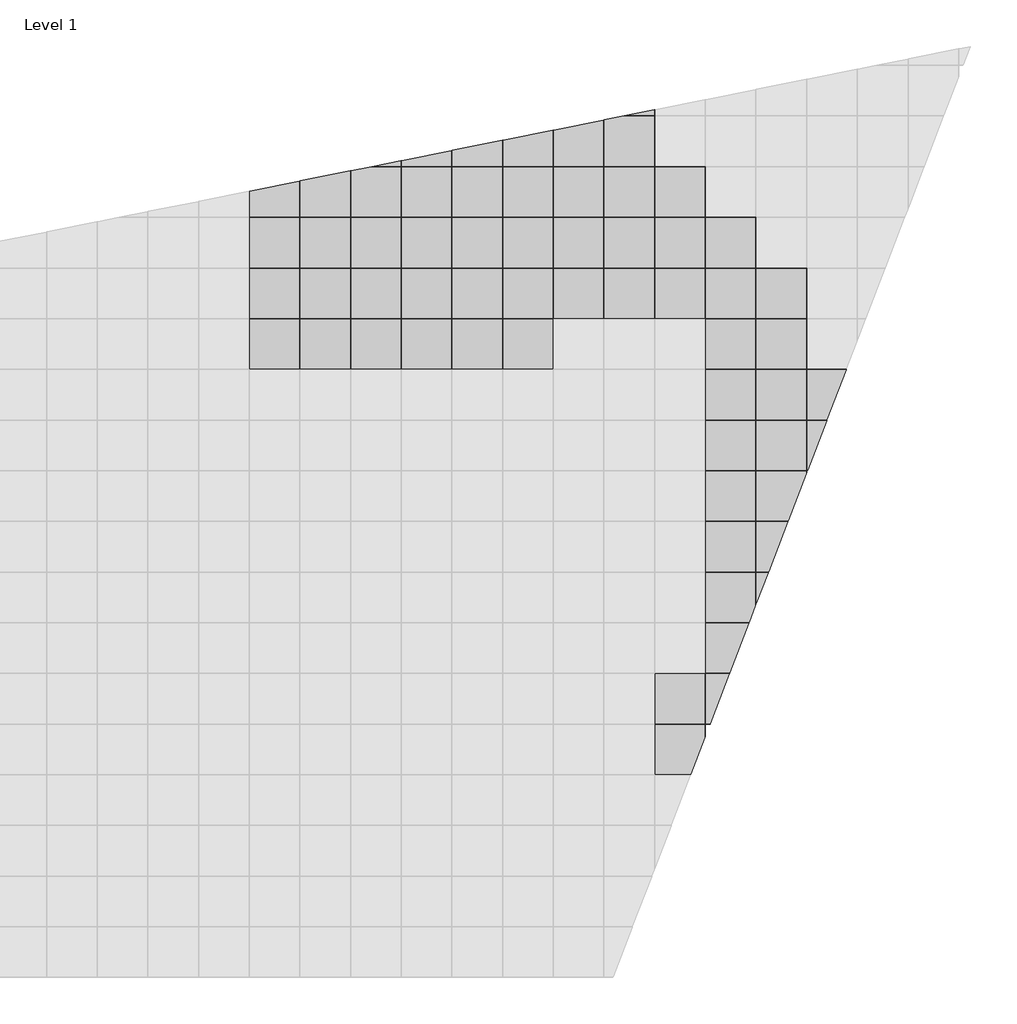
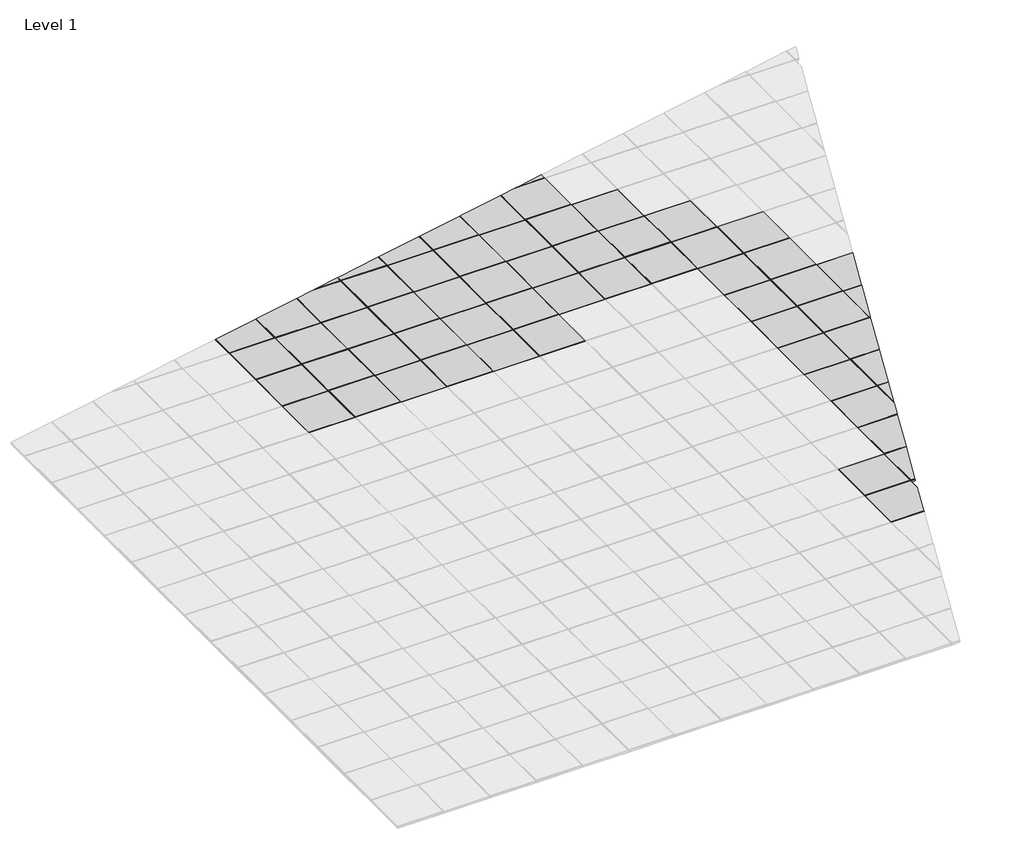
# One storey, part 7 of 18: 61 plates.
"""IFC4 building model written with IfcOpenShell, lengths in millimetres."""

import ifcopenshell
import ifcopenshell.guid

model = None  # the IFC model being written
_history = None  # IfcOwnerHistory: only IFC2X3 demands one
_inside = {}  # id of a spatial element -> (the spatial element, [elements in it])
_under = {}  # id of a project, library or spatial element -> (it, [spatial elements below it])
_declared = {}  # id of a project -> (the project, [libraries it declares])
_typed = {}  # id of a type object -> (the type object, [elements of that type])
_made_of = {}  # id of a material, layer set ... -> (it, [elements and type objects made of it])


def new_model(schema):
    """Start an empty IFC model of exactly this schema.

    Asked for "IFC4X3", IfcOpenShell would pick the latest addendum, in which some entities
    have other attributes; the version numbers below select the first issue.
    IFC2X3 requires an IfcOwnerHistory on every rooted entity: one is made here for all.
    """
    global model, _history
    if schema == "IFC4X3":
        model = ifcopenshell.file(schema_version=(4, 3, 0, 0))
    else:
        model = ifcopenshell.file(schema=schema)
    _inside.clear()
    _under.clear()
    _declared.clear()
    _typed.clear()
    _made_of.clear()
    _history = None
    if model.schema == "IFC2X3":
        org = make("IfcOrganization", Name="unknown")
        user = make(
            "IfcPersonAndOrganization",
            ThePerson=make("IfcPerson", FamilyName="unknown"),
            TheOrganization=org,
        )
        app = make(
            "IfcApplication",
            ApplicationDeveloper=org,
            Version="unknown",
            ApplicationFullName="unknown",
            ApplicationIdentifier="unknown",
        )
        _history = make(
            "IfcOwnerHistory",
            OwningUser=user,
            OwningApplication=app,
            ChangeAction="ADDED",
            CreationDate=0,
        )
    return model


def make(cls, **values):
    """One entity of the class cls with the attributes given. An attribute that is None is left unset."""
    return model.create_entity(
        cls, **{name: value for name, value in values.items() if value is not None}
    )


def rooted(cls, **values):
    """An entity with a GlobalId (a new one), such as an element, a storey or a relation."""
    return make(cls, GlobalId=ifcopenshell.guid.new(), OwnerHistory=_history, **values)


def si_unit(unit_type, name, prefix=None):
    """IfcSIUnit, for example si_unit("LENGTHUNIT", "METRE", prefix="MILLI")."""
    return make("IfcSIUnit", UnitType=unit_type, Prefix=prefix, Name=name)


def assignment(units):
    """IfcUnitAssignment: the units of a project."""
    return None if units is None else make("IfcUnitAssignment", Units=units)


def point(xyz):
    """IfcCartesianPoint."""
    return None if xyz is None else make("IfcCartesianPoint", Coordinates=xyz)


def direction(xyz):
    """IfcDirection."""
    return None if xyz is None else make("IfcDirection", DirectionRatios=xyz)


def frame(location, z_axis=None, x_axis=None):
    """IfcAxis2Placement3D, a coordinate frame: its origin and axes. An axis left out is left unset."""
    return make(
        "IfcAxis2Placement3D",
        Location=point(location),
        Axis=direction(z_axis),
        RefDirection=direction(x_axis),
    )


def origin():
    """The frame at (0, 0, 0) with its axes left unset."""
    return frame((0.0, 0.0, 0.0))


def origin_with_axes():
    """The frame at (0, 0, 0) with the z axis (0, 0, 1) and the x axis (1, 0, 0) written out."""
    return frame((0.0, 0.0, 0.0), z_axis=(0.0, 0.0, 1.0), x_axis=(1.0, 0.0, 0.0))


def place(relative_to, where):
    """IfcLocalPlacement: puts the frame where relative to a parent placement (None: the world)."""
    return make(
        "IfcLocalPlacement", PlacementRelTo=relative_to, RelativePlacement=where
    )


def context(
    kind, dimensions, precision=None, world=None, true_north=None, identifier=None
):
    """IfcGeometricRepresentationContext, for example the 3D "Model" context."""
    return make(
        "IfcGeometricRepresentationContext",
        ContextIdentifier=identifier,
        ContextType=kind,
        CoordinateSpaceDimension=dimensions,
        Precision=precision,
        WorldCoordinateSystem=world,
        TrueNorth=true_north,
    )


def project(units=None, contexts=None):
    """IfcProject with its units and contexts."""
    return rooted(
        "IfcProject",
        Name="project",
        RepresentationContexts=contexts,
        UnitsInContext=assignment(units),
    )


def spatial(cls, under=None, at=None, **own):
    """A site, building, storey or space (cls), placed at a placement, below another one or the project."""
    s = rooted(cls, ObjectPlacement=at, **own)
    if under is not None:
        _under.setdefault(under.id(), (under, []))[1].append(s)
    return s


def polyline(points):
    """IfcPolyline through the points."""
    return make("IfcPolyline", Points=[point(p) for p in points])


def outline(outer, holes=None, kind="AREA"):
    """IfcArbitraryClosedProfileDef: a profile drawn as a closed curve; with holes, ...WithVoids."""
    if holes is None:
        return make("IfcArbitraryClosedProfileDef", ProfileType=kind, OuterCurve=outer)
    return make(
        "IfcArbitraryProfileDefWithVoids",
        ProfileType=kind,
        OuterCurve=outer,
        InnerCurves=holes,
    )


def extrude(swept, where, along, depth):
    """IfcExtrudedAreaSolid: the profile swept, set in the frame where, extruded along a direction by depth."""
    return make(
        "IfcExtrudedAreaSolid",
        SweptArea=swept,
        Position=where,
        ExtrudedDirection=direction(along),
        Depth=depth,
    )


def shape(context_of_items, identifier, shape_type, items):
    """IfcShapeRepresentation: the items that make up one representation, for example the "Body"."""
    return make(
        "IfcShapeRepresentation",
        ContextOfItems=context_of_items,
        RepresentationIdentifier=identifier,
        RepresentationType=shape_type,
        Items=items,
    )


def source(mapping_origin, context_of_items, identifier, shape_type, items):
    """IfcRepresentationMap: a shape defined once, which mapped items show again and again."""
    return make(
        "IfcRepresentationMap",
        MappingOrigin=mapping_origin,
        MappedRepresentation=shape(context_of_items, identifier, shape_type, items),
    )


def transform(
    local_origin,
    x_axis=None,
    y_axis=None,
    z_axis=None,
    scale=None,
    scale2=None,
    scale3=None,
    uniform=True,
):
    """IfcCartesianTransformationOperator3D, or its non-uniform kind. x_axis, y_axis, z_axis: its Axis1, 2, 3."""
    if uniform:
        return make(
            "IfcCartesianTransformationOperator3D",
            Axis1=direction(x_axis),
            Axis2=direction(y_axis),
            LocalOrigin=point(local_origin),
            Scale=scale,
            Axis3=direction(z_axis),
        )
    return make(
        "IfcCartesianTransformationOperator3DnonUniform",
        Axis1=direction(x_axis),
        Axis2=direction(y_axis),
        LocalOrigin=point(local_origin),
        Scale=scale,
        Axis3=direction(z_axis),
        Scale2=scale2,
        Scale3=scale3,
    )


def mapped(mapping_source, mapping_target):
    """IfcMappedItem: shows the shape of a source again, moved by a transform."""
    return make(
        "IfcMappedItem", MappingSource=mapping_source, MappingTarget=mapping_target
    )


def made_of(thing, what):
    """Note that an element or type object is made of a material, layer set ...; save() writes the relation."""
    if what is not None:
        _made_of.setdefault(what.id(), (what, []))[1].append(thing)
    return thing


def element(
    cls,
    number,
    at=None,
    inside=None,
    cuts=None,
    type_object=None,
    material=None,
    context=None,
    identifier="Body",
    shape_type=None,
    held_by="IfcProductDefinitionShape",
    body=None,
    shapes=None,
    **own,
):
    """One element of the class cls, such as IfcWall. Its Tag is "e" and its number.

    at: its placement. inside: the storey or other place that contains it. cuts: it is an
    opening in that element (IfcRelVoidsElement). A single representation is given by context,
    identifier, shape_type and body (its items); several are given by shapes. held_by: the class
    of the entity that holds the representations. save() writes the other relations.
    """
    e = rooted(cls, Tag="e%d" % number, ObjectPlacement=at, **own)
    if body is not None:
        shapes = [shape(context, identifier, shape_type, body)]
    if shapes is not None:
        e.Representation = make(held_by, Representations=shapes)
    if inside is not None:
        _inside.setdefault(inside.id(), (inside, []))[1].append(e)
    if cuts is not None:
        rooted(
            "IfcRelVoidsElement", RelatingBuildingElement=cuts, RelatedOpeningElement=e
        )
    if type_object is not None:
        _typed.setdefault(type_object.id(), (type_object, []))[1].append(e)
    return made_of(e, material)


def aggregate(whole, parts):
    """IfcRelAggregates: a whole, such as a stair, and the parts it consists of."""
    return rooted("IfcRelAggregates", RelatingObject=whole, RelatedObjects=parts)


def save(model, path):
    """Write the relations noted so far, then the file.

    IfcRelAggregates (storeys below a building ...), IfcRelContainedInSpatialStructure (elements
    in a storey), IfcRelDefinesByType, IfcRelAssociatesMaterial and IfcRelDeclares: one each for
    every whole, place, type object, material and project.
    """
    for whole, parts in _under.values():
        aggregate(whole, parts)
    for where, things in _inside.values():
        rooted(
            "IfcRelContainedInSpatialStructure",
            RelatedElements=things,
            RelatingStructure=where,
        )
    for kind, things in _typed.values():
        rooted("IfcRelDefinesByType", RelatedObjects=things, RelatingType=kind)
    for what, things in _made_of.values():
        rooted("IfcRelAssociatesMaterial", RelatedObjects=things, RelatingMaterial=what)
    for by, libraries in _declared.values():
        rooted("IfcRelDeclares", RelatingContext=by, RelatedDefinitions=libraries)
    model.write(path)


def type_1_8eb2385c(model_context):
    return source(origin(), model_context, "Body", "SweptSolid", [
        extrude(outline(polyline([(1000.0, 500.0), (500.0, 500.0), (500.0, 1000.0), (1000.0, 1000.0), (1000.0, 500.0)]), holes=[polyline([(995.0, 995.0), (505.0, 995.0), (505.0, 505.0), (995.0, 505.0), (995.0, 995.0)])]), origin_with_axes(), (0.0, 0.0, 1.0), 18.0),
        extrude(outline(polyline([(505.0, 995.0), (995.0, 995.0), (995.0, 505.0), (505.0, 505.0), (505.0, 995.0)])), origin_with_axes(), (0.0, 0.0, 1.0), 20.0),
    ])


model = new_model("IFC4")

# Units and contexts
model_context = context("Model", 3, world=origin())
ifc_project = project(units=[si_unit("LENGTHUNIT", "METRE", prefix="MILLI")], contexts=[model_context])

# Site, building, storey
site = spatial("IfcSite", under=ifc_project)
building = spatial("IfcBuilding", under=site)
storey = spatial("IfcBuildingStorey", under=building, Name="Level 1", Elevation=0.0)

# Plates
placement = place(None, origin())
element("IfcPlate", 1, ObjectType="00_CPA_tegel : Type 1", at=placement, inside=storey, context=model_context, shape_type="SweptSolid", body=[
    extrude(outline(polyline([(16011.2147669, 16097.7016515), (16011.2147669, 16587.7016515), (16501.2147669, 16587.7016515), (16501.2147669, 16456.8505515), (16363.3882861, 16097.7016515), (16011.2147669, 16097.7016515)])), origin_with_axes(), (0.0, 0.0, 1.0), 20.0),
    extrude(outline(polyline([(16006.2147669, 16592.7016515), (16506.2147669, 16592.7016515), (16506.2147669, 16469.8795753), (16501.2147669, 16456.8505515), (16501.2147669, 16587.7016515), (16011.2147669, 16587.7016515), (16011.2147669, 16097.7016515), (16363.3882861, 16097.7016515), (16361.4694931, 16092.7016515), (16006.2147669, 16092.7016515), (16006.2147669, 16592.7016515)])), origin_with_axes(), (0.0, 0.0, 1.0), 18.0),
])
element("IfcPlate", 2, ObjectType="00_CPA_tegel : Type 1", at=placement, inside=storey, context=model_context, shape_type="SweptSolid", body=[
    extrude(outline(polyline([(16011.2147669, 16597.7016515), (16011.2147669, 17087.7016515), (16501.2147669, 17087.7016515), (16501.2147669, 16597.7016515), (16011.2147669, 16597.7016515)])), origin_with_axes(), (0.0, 0.0, 1.0), 20.0),
    extrude(outline(polyline([(16506.2147669, 16592.7016515), (16006.2147669, 16592.7016515), (16006.2147669, 17092.7016515), (16506.2147669, 17092.7016515), (16506.2147669, 16592.7016515)]), holes=[polyline([(16501.2147669, 17087.7016515), (16011.2147669, 17087.7016515), (16011.2147669, 16597.7016515), (16501.2147669, 16597.7016515), (16501.2147669, 17087.7016515)])]), origin_with_axes(), (0.0, 0.0, 1.0), 18.0),
])
element("IfcPlate", 3, ObjectType="00_CPA_tegel : Type 1", at=placement, inside=storey, context=model_context, shape_type="SweptSolid", body=[
    extrude(outline(polyline([(16511.2147669, 16597.7016515), (16511.2147669, 17087.7016515), (16743.3093049, 17087.7016515), (16555.2675885, 16597.7016515), (16511.2147669, 16597.7016515)])), origin_with_axes(), (0.0, 0.0, 1.0), 20.0),
    extrude(outline(polyline([(16506.2147669, 16592.7016515), (16506.2147669, 17092.7016515), (16745.2280979, 17092.7016515), (16743.3093049, 17087.7016515), (16511.2147669, 17087.7016515), (16511.2147669, 16597.7016515), (16555.2675885, 16597.7016515), (16553.3487955, 16592.7016515), (16506.2147669, 16592.7016515)])), origin_with_axes(), (0.0, 0.0, 1.0), 18.0),
])
element("IfcPlate", 4, ObjectType="00_CPA_tegel : Type 1", at=placement, inside=storey, context=model_context, shape_type="SweptSolid", body=[
    extrude(outline(polyline([(16511.2147669, 17097.7016515), (16511.2147669, 17587.7016515), (16935.1886073, 17587.7016515), (16747.146891, 17097.7016515), (16511.2147669, 17097.7016515)])), origin_with_axes(), (0.0, 0.0, 1.0), 20.0),
    extrude(outline(polyline([(16506.2147669, 17092.7016515), (16506.2147669, 17592.7016515), (16937.1074003, 17592.7016515), (16935.1886073, 17587.7016515), (16511.2147669, 17587.7016515), (16511.2147669, 17097.7016515), (16747.146891, 17097.7016515), (16745.2280979, 17092.7016515), (16506.2147669, 17092.7016515)])), origin_with_axes(), (0.0, 0.0, 1.0), 18.0),
])
element("IfcPlate", 5, ObjectType="00_CPA_tegel : Type 1", at=placement, inside=storey, context=model_context, shape_type="SweptSolid", body=[
    extrude(outline(polyline([(16511.2147669, 17597.7016515), (16511.2147669, 18087.7016515), (17001.2147669, 18087.7016515), (17001.2147669, 17759.7529326), (16939.0261934, 17597.7016515), (16511.2147669, 17597.7016515)])), origin_with_axes(), (0.0, 0.0, 1.0), 20.0),
    extrude(outline(polyline([(16506.2147669, 18092.7016515), (17006.2147669, 18092.7016515), (17006.2147669, 17772.7819564), (17001.2147669, 17759.7529326), (17001.2147669, 18087.7016515), (16511.2147669, 18087.7016515), (16511.2147669, 17597.7016515), (16939.0261934, 17597.7016515), (16937.1074003, 17592.7016515), (16506.2147669, 17592.7016515), (16506.2147669, 18092.7016515)])), origin_with_axes(), (0.0, 0.0, 1.0), 18.0),
])
element("IfcPlate", 6, ObjectType="00_CPA_tegel : Type 1", at=placement, inside=storey, context=model_context, shape_type="SweptSolid", body=[
    extrude(outline(polyline([(17011.2147669, 17785.8109803), (17011.2147669, 18087.7016515), (17127.0679097, 18087.7016515), (17011.2147669, 17785.8109803)])), origin_with_axes(), (0.0, 0.0, 1.0), 20.0),
    extrude(outline(polyline([(17006.2147669, 18092.7016515), (17128.9867027, 18092.7016515), (17127.0679097, 18087.7016515), (17011.2147669, 18087.7016515), (17011.2147669, 17785.8109803), (17006.2147669, 17772.7819564), (17006.2147669, 18092.7016515)])), origin_with_axes(), (0.0, 0.0, 1.0), 18.0),
])
element("IfcPlate", 7, ObjectType="00_CPA_tegel : Type 1", at=placement, inside=storey, context=model_context, shape_type="SweptSolid", body=[
    extrude(outline(polyline([(17011.2147669, 18097.7016515), (17011.2147669, 18587.7016515), (17318.9472121, 18587.7016515), (17130.9054958, 18097.7016515), (17011.2147669, 18097.7016515)])), origin_with_axes(), (0.0, 0.0, 1.0), 20.0),
    extrude(outline(polyline([(17006.2147669, 18092.7016515), (17006.2147669, 18592.7016515), (17320.8660051, 18592.7016515), (17318.9472121, 18587.7016515), (17011.2147669, 18587.7016515), (17011.2147669, 18097.7016515), (17130.9054958, 18097.7016515), (17128.9867027, 18092.7016515), (17006.2147669, 18092.7016515)])), origin_with_axes(), (0.0, 0.0, 1.0), 18.0),
])
element("IfcPlate", 8, ObjectType="00_CPA_tegel : Type 1", at=placement, inside=storey, context=model_context, shape_type="SweptSolid", body=[
    extrude(outline(polyline([(17011.2147669, 18597.7016515), (17011.2147669, 19087.7016515), (17501.2147669, 19087.7016515), (17501.2147669, 19062.6553138), (17322.7847982, 18597.7016515), (17011.2147669, 18597.7016515)])), origin_with_axes(), (0.0, 0.0, 1.0), 20.0),
    extrude(outline(polyline([(17006.2147669, 19092.7016515), (17506.2147669, 19092.7016515), (17506.2147669, 19075.6843376), (17501.2147669, 19062.6553138), (17501.2147669, 19087.7016515), (17011.2147669, 19087.7016515), (17011.2147669, 18597.7016515), (17322.7847982, 18597.7016515), (17320.8660051, 18592.7016515), (17006.2147669, 18592.7016515), (17006.2147669, 19092.7016515)])), origin_with_axes(), (0.0, 0.0, 1.0), 18.0),
])
element("IfcPlate", 9, ObjectType="00_CPA_tegel : Type 1", at=placement, inside=storey, context=model_context, shape_type="SweptSolid", body=[
    extrude(outline(polyline([(17011.2147669, 19097.7016515), (17011.2147669, 19587.7016515), (17501.2147669, 19587.7016515), (17501.2147669, 19097.7016515), (17011.2147669, 19097.7016515)])), origin_with_axes(), (0.0, 0.0, 1.0), 20.0),
    extrude(outline(polyline([(17506.2147669, 19092.7016515), (17006.2147669, 19092.7016515), (17006.2147669, 19592.7016515), (17506.2147669, 19592.7016515), (17506.2147669, 19092.7016515)]), holes=[polyline([(17501.2147669, 19587.7016515), (17011.2147669, 19587.7016515), (17011.2147669, 19097.7016515), (17501.2147669, 19097.7016515), (17501.2147669, 19587.7016515)])]), origin_with_axes(), (0.0, 0.0, 1.0), 18.0),
])
element("IfcPlate", 10, ObjectType="00_CPA_tegel : Type 1", at=placement, inside=storey, context=model_context, shape_type="SweptSolid", body=[
    extrude(outline(polyline([(17511.2147669, 19097.7016515), (17511.2147669, 19587.7016515), (17702.7058169, 19587.7016515), (17514.6641006, 19097.7016515), (17511.2147669, 19097.7016515)])), origin_with_axes(), (0.0, 0.0, 1.0), 20.0),
    extrude(outline(polyline([(17506.2147669, 19092.7016515), (17506.2147669, 19592.7016515), (17704.62461, 19592.7016515), (17702.7058169, 19587.7016515), (17511.2147669, 19587.7016515), (17511.2147669, 19097.7016515), (17514.6641006, 19097.7016515), (17512.7453076, 19092.7016515), (17506.2147669, 19092.7016515)])), origin_with_axes(), (0.0, 0.0, 1.0), 18.0),
])
element("IfcPlate", 11, ObjectType="00_CPA_tegel : Type 1", at=placement, inside=storey, context=model_context, shape_type="SweptSolid", body=[
    extrude(outline(polyline([(17511.2147669, 19597.7016515), (17511.2147669, 20087.7016515), (17894.5851193, 20087.7016515), (17706.543403, 19597.7016515), (17511.2147669, 19597.7016515)])), origin_with_axes(), (0.0, 0.0, 1.0), 20.0),
    extrude(outline(polyline([(17506.2147669, 19592.7016515), (17506.2147669, 20092.7016515), (17896.5039124, 20092.7016515), (17894.5851193, 20087.7016515), (17511.2147669, 20087.7016515), (17511.2147669, 19597.7016515), (17706.543403, 19597.7016515), (17704.62461, 19592.7016515), (17506.2147669, 19592.7016515)])), origin_with_axes(), (0.0, 0.0, 1.0), 18.0),
])
element("IfcPlate", 12, ObjectType="00_CPA_tegel : Type 1", at=placement, inside=storey, context=model_context, shape_type="SweptSolid", body=[
    extrude(outline(polyline([(12011.2147669, 20587.7016515), (12501.2147669, 20587.7016515), (12501.2147669, 20097.7016515), (12011.2147669, 20097.7016515), (12011.2147669, 20587.7016515)])), origin_with_axes(), (0.0, 0.0, 1.0), 20.0),
    extrude(outline(polyline([(12506.2147669, 20092.7016515), (12006.2147669, 20092.7016515), (12006.2147669, 20592.7016515), (12506.2147669, 20592.7016515), (12506.2147669, 20092.7016515)]), holes=[polyline([(12501.2147669, 20587.7016515), (12011.2147669, 20587.7016515), (12011.2147669, 20097.7016515), (12501.2147669, 20097.7016515), (12501.2147669, 20587.7016515)])]), origin_with_axes(), (0.0, 0.0, 1.0), 18.0),
])
element("IfcPlate", 13, ObjectType="00_CPA_tegel : Type 1", at=placement, inside=storey, context=model_context, shape_type="SweptSolid", body=[
    extrude(outline(polyline([(12511.2147669, 20587.7016515), (13001.2147669, 20587.7016515), (13001.2147669, 20097.7016515), (12511.2147669, 20097.7016515), (12511.2147669, 20587.7016515)])), origin_with_axes(), (0.0, 0.0, 1.0), 20.0),
    extrude(outline(polyline([(13006.2147669, 20092.7016515), (12506.2147669, 20092.7016515), (12506.2147669, 20592.7016515), (13006.2147669, 20592.7016515), (13006.2147669, 20092.7016515)]), holes=[polyline([(13001.2147669, 20587.7016515), (12511.2147669, 20587.7016515), (12511.2147669, 20097.7016515), (13001.2147669, 20097.7016515), (13001.2147669, 20587.7016515)])]), origin_with_axes(), (0.0, 0.0, 1.0), 18.0),
])
element("IfcPlate", 14, ObjectType="00_CPA_tegel : Type 1", at=placement, inside=storey, context=model_context, shape_type="SweptSolid", body=[
    extrude(outline(polyline([(13011.2147669, 20587.7016515), (13501.2147669, 20587.7016515), (13501.2147669, 20097.7016515), (13011.2147669, 20097.7016515), (13011.2147669, 20587.7016515)])), origin_with_axes(), (0.0, 0.0, 1.0), 20.0),
    extrude(outline(polyline([(13506.2147669, 20092.7016515), (13006.2147669, 20092.7016515), (13006.2147669, 20592.7016515), (13506.2147669, 20592.7016515), (13506.2147669, 20092.7016515)]), holes=[polyline([(13501.2147669, 20587.7016515), (13011.2147669, 20587.7016515), (13011.2147669, 20097.7016515), (13501.2147669, 20097.7016515), (13501.2147669, 20587.7016515)])]), origin_with_axes(), (0.0, 0.0, 1.0), 18.0),
])
element("IfcPlate", 15, ObjectType="00_CPA_tegel : Type 1", at=placement, inside=storey, context=model_context, shape_type="SweptSolid", body=[
    extrude(outline(polyline([(13511.2147669, 20587.7016515), (14001.2147669, 20587.7016515), (14001.2147669, 20097.7016515), (13511.2147669, 20097.7016515), (13511.2147669, 20587.7016515)])), origin_with_axes(), (0.0, 0.0, 1.0), 20.0),
    extrude(outline(polyline([(14006.2147669, 20092.7016515), (13506.2147669, 20092.7016515), (13506.2147669, 20592.7016515), (14006.2147669, 20592.7016515), (14006.2147669, 20092.7016515)]), holes=[polyline([(14001.2147669, 20587.7016515), (13511.2147669, 20587.7016515), (13511.2147669, 20097.7016515), (14001.2147669, 20097.7016515), (14001.2147669, 20587.7016515)])]), origin_with_axes(), (0.0, 0.0, 1.0), 18.0),
])
element("IfcPlate", 16, ObjectType="00_CPA_tegel : Type 1", at=placement, inside=storey, context=model_context, shape_type="SweptSolid", body=[
    extrude(outline(polyline([(14011.2147669, 20587.7016515), (14501.2147669, 20587.7016515), (14501.2147669, 20097.7016515), (14011.2147669, 20097.7016515), (14011.2147669, 20587.7016515)])), origin_with_axes(), (0.0, 0.0, 1.0), 20.0),
    extrude(outline(polyline([(14506.2147669, 20092.7016515), (14006.2147669, 20092.7016515), (14006.2147669, 20592.7016515), (14506.2147669, 20592.7016515), (14506.2147669, 20092.7016515)]), holes=[polyline([(14501.2147669, 20587.7016515), (14011.2147669, 20587.7016515), (14011.2147669, 20097.7016515), (14501.2147669, 20097.7016515), (14501.2147669, 20587.7016515)])]), origin_with_axes(), (0.0, 0.0, 1.0), 18.0),
])
element("IfcPlate", 17, ObjectType="00_CPA_tegel : Type 1", at=placement, inside=storey, context=model_context, shape_type="SweptSolid", body=[
    extrude(outline(polyline([(14511.2147669, 20587.7016515), (15001.2147669, 20587.7016515), (15001.2147669, 20097.7016515), (14511.2147669, 20097.7016515), (14511.2147669, 20587.7016515)])), origin_with_axes(), (0.0, 0.0, 1.0), 20.0),
    extrude(outline(polyline([(15006.2147669, 20092.7016515), (14506.2147669, 20092.7016515), (14506.2147669, 20592.7016515), (15006.2147669, 20592.7016515), (15006.2147669, 20092.7016515)]), holes=[polyline([(15001.2147669, 20587.7016515), (14511.2147669, 20587.7016515), (14511.2147669, 20097.7016515), (15001.2147669, 20097.7016515), (15001.2147669, 20587.7016515)])]), origin_with_axes(), (0.0, 0.0, 1.0), 18.0),
])
element("IfcPlate", 18, ObjectType="00_CPA_tegel : Type 1", at=placement, inside=storey, context=model_context, shape_type="SweptSolid", body=[
    extrude(outline(polyline([(12011.2147669, 21087.7016515), (12501.2147669, 21087.7016515), (12501.2147669, 20597.7016515), (12011.2147669, 20597.7016515), (12011.2147669, 21087.7016515)])), origin_with_axes(), (0.0, 0.0, 1.0), 20.0),
    extrude(outline(polyline([(12506.2147669, 20592.7016515), (12006.2147669, 20592.7016515), (12006.2147669, 21092.7016515), (12506.2147669, 21092.7016515), (12506.2147669, 20592.7016515)]), holes=[polyline([(12501.2147669, 21087.7016515), (12011.2147669, 21087.7016515), (12011.2147669, 20597.7016515), (12501.2147669, 20597.7016515), (12501.2147669, 21087.7016515)])]), origin_with_axes(), (0.0, 0.0, 1.0), 18.0),
])
element("IfcPlate", 19, ObjectType="00_CPA_tegel : Type 1", at=placement, inside=storey, context=model_context, shape_type="SweptSolid", body=[
    extrude(outline(polyline([(12511.2147669, 21087.7016515), (13001.2147669, 21087.7016515), (13001.2147669, 20597.7016515), (12511.2147669, 20597.7016515), (12511.2147669, 21087.7016515)])), origin_with_axes(), (0.0, 0.0, 1.0), 20.0),
    extrude(outline(polyline([(13006.2147669, 20592.7016515), (12506.2147669, 20592.7016515), (12506.2147669, 21092.7016515), (13006.2147669, 21092.7016515), (13006.2147669, 20592.7016515)]), holes=[polyline([(13001.2147669, 21087.7016515), (12511.2147669, 21087.7016515), (12511.2147669, 20597.7016515), (13001.2147669, 20597.7016515), (13001.2147669, 21087.7016515)])]), origin_with_axes(), (0.0, 0.0, 1.0), 18.0),
])
element("IfcPlate", 20, ObjectType="00_CPA_tegel : Type 1", at=placement, inside=storey, context=model_context, shape_type="SweptSolid", body=[
    extrude(outline(polyline([(13011.2147669, 21087.7016515), (13501.2147669, 21087.7016515), (13501.2147669, 20597.7016515), (13011.2147669, 20597.7016515), (13011.2147669, 21087.7016515)])), origin_with_axes(), (0.0, 0.0, 1.0), 20.0),
    extrude(outline(polyline([(13506.2147669, 20592.7016515), (13006.2147669, 20592.7016515), (13006.2147669, 21092.7016515), (13506.2147669, 21092.7016515), (13506.2147669, 20592.7016515)]), holes=[polyline([(13501.2147669, 21087.7016515), (13011.2147669, 21087.7016515), (13011.2147669, 20597.7016515), (13501.2147669, 20597.7016515), (13501.2147669, 21087.7016515)])]), origin_with_axes(), (0.0, 0.0, 1.0), 18.0),
])
element("IfcPlate", 21, ObjectType="00_CPA_tegel : Type 1", at=placement, inside=storey, context=model_context, shape_type="SweptSolid", body=[
    extrude(outline(polyline([(13511.2147669, 21087.7016515), (14001.2147669, 21087.7016515), (14001.2147669, 20597.7016515), (13511.2147669, 20597.7016515), (13511.2147669, 21087.7016515)])), origin_with_axes(), (0.0, 0.0, 1.0), 20.0),
    extrude(outline(polyline([(14006.2147669, 20592.7016515), (13506.2147669, 20592.7016515), (13506.2147669, 21092.7016515), (14006.2147669, 21092.7016515), (14006.2147669, 20592.7016515)]), holes=[polyline([(14001.2147669, 21087.7016515), (13511.2147669, 21087.7016515), (13511.2147669, 20597.7016515), (14001.2147669, 20597.7016515), (14001.2147669, 21087.7016515)])]), origin_with_axes(), (0.0, 0.0, 1.0), 18.0),
])
element("IfcPlate", 22, ObjectType="00_CPA_tegel : Type 1", at=placement, inside=storey, context=model_context, shape_type="SweptSolid", body=[
    extrude(outline(polyline([(14011.2147669, 21087.7016515), (14501.2147669, 21087.7016515), (14501.2147669, 20597.7016515), (14011.2147669, 20597.7016515), (14011.2147669, 21087.7016515)])), origin_with_axes(), (0.0, 0.0, 1.0), 20.0),
    extrude(outline(polyline([(14506.2147669, 20592.7016515), (14006.2147669, 20592.7016515), (14006.2147669, 21092.7016515), (14506.2147669, 21092.7016515), (14506.2147669, 20592.7016515)]), holes=[polyline([(14501.2147669, 21087.7016515), (14011.2147669, 21087.7016515), (14011.2147669, 20597.7016515), (14501.2147669, 20597.7016515), (14501.2147669, 21087.7016515)])]), origin_with_axes(), (0.0, 0.0, 1.0), 18.0),
])
element("IfcPlate", 23, ObjectType="00_CPA_tegel : Type 1", at=placement, inside=storey, context=model_context, shape_type="SweptSolid", body=[
    extrude(outline(polyline([(14511.2147669, 21087.7016515), (15001.2147669, 21087.7016515), (15001.2147669, 20597.7016515), (14511.2147669, 20597.7016515), (14511.2147669, 21087.7016515)])), origin_with_axes(), (0.0, 0.0, 1.0), 20.0),
    extrude(outline(polyline([(15006.2147669, 20592.7016515), (14506.2147669, 20592.7016515), (14506.2147669, 21092.7016515), (15006.2147669, 21092.7016515), (15006.2147669, 20592.7016515)]), holes=[polyline([(15001.2147669, 21087.7016515), (14511.2147669, 21087.7016515), (14511.2147669, 20597.7016515), (15001.2147669, 20597.7016515), (15001.2147669, 21087.7016515)])]), origin_with_axes(), (0.0, 0.0, 1.0), 18.0),
])
element("IfcPlate", 24, ObjectType="00_CPA_tegel : Type 1", at=placement, inside=storey, context=model_context, shape_type="SweptSolid", body=[
    extrude(outline(polyline([(12011.2147669, 21587.7016515), (12501.2147669, 21587.7016515), (12501.2147669, 21097.7016515), (12011.2147669, 21097.7016515), (12011.2147669, 21587.7016515)])), origin_with_axes(), (0.0, 0.0, 1.0), 20.0),
    extrude(outline(polyline([(12506.2147669, 21092.7016515), (12006.2147669, 21092.7016515), (12006.2147669, 21592.7016515), (12506.2147669, 21592.7016515), (12506.2147669, 21092.7016515)]), holes=[polyline([(12501.2147669, 21587.7016515), (12011.2147669, 21587.7016515), (12011.2147669, 21097.7016515), (12501.2147669, 21097.7016515), (12501.2147669, 21587.7016515)])]), origin_with_axes(), (0.0, 0.0, 1.0), 18.0),
])
element("IfcPlate", 25, ObjectType="00_CPA_tegel : Type 1", at=placement, inside=storey, context=model_context, shape_type="SweptSolid", body=[
    extrude(outline(polyline([(12511.2147669, 21587.7016515), (13001.2147669, 21587.7016515), (13001.2147669, 21097.7016515), (12511.2147669, 21097.7016515), (12511.2147669, 21587.7016515)])), origin_with_axes(), (0.0, 0.0, 1.0), 20.0),
    extrude(outline(polyline([(13006.2147669, 21092.7016515), (12506.2147669, 21092.7016515), (12506.2147669, 21592.7016515), (13006.2147669, 21592.7016515), (13006.2147669, 21092.7016515)]), holes=[polyline([(13001.2147669, 21587.7016515), (12511.2147669, 21587.7016515), (12511.2147669, 21097.7016515), (13001.2147669, 21097.7016515), (13001.2147669, 21587.7016515)])]), origin_with_axes(), (0.0, 0.0, 1.0), 18.0),
])
element("IfcPlate", 26, ObjectType="00_CPA_tegel : Type 1", at=placement, inside=storey, context=model_context, shape_type="SweptSolid", body=[
    extrude(outline(polyline([(13011.2147669, 21587.7016515), (13501.2147669, 21587.7016515), (13501.2147669, 21097.7016515), (13011.2147669, 21097.7016515), (13011.2147669, 21587.7016515)])), origin_with_axes(), (0.0, 0.0, 1.0), 20.0),
    extrude(outline(polyline([(13506.2147669, 21092.7016515), (13006.2147669, 21092.7016515), (13006.2147669, 21592.7016515), (13506.2147669, 21592.7016515), (13506.2147669, 21092.7016515)]), holes=[polyline([(13501.2147669, 21587.7016515), (13011.2147669, 21587.7016515), (13011.2147669, 21097.7016515), (13501.2147669, 21097.7016515), (13501.2147669, 21587.7016515)])]), origin_with_axes(), (0.0, 0.0, 1.0), 18.0),
])
element("IfcPlate", 27, ObjectType="00_CPA_tegel : Type 1", at=placement, inside=storey, context=model_context, shape_type="SweptSolid", body=[
    extrude(outline(polyline([(13511.2147669, 21587.7016515), (14001.2147669, 21587.7016515), (14001.2147669, 21097.7016515), (13511.2147669, 21097.7016515), (13511.2147669, 21587.7016515)])), origin_with_axes(), (0.0, 0.0, 1.0), 20.0),
    extrude(outline(polyline([(14006.2147669, 21092.7016515), (13506.2147669, 21092.7016515), (13506.2147669, 21592.7016515), (14006.2147669, 21592.7016515), (14006.2147669, 21092.7016515)]), holes=[polyline([(14001.2147669, 21587.7016515), (13511.2147669, 21587.7016515), (13511.2147669, 21097.7016515), (14001.2147669, 21097.7016515), (14001.2147669, 21587.7016515)])]), origin_with_axes(), (0.0, 0.0, 1.0), 18.0),
])
element("IfcPlate", 28, ObjectType="00_CPA_tegel : Type 1", at=placement, inside=storey, context=model_context, shape_type="SweptSolid", body=[
    extrude(outline(polyline([(14011.2147669, 21587.7016515), (14501.2147669, 21587.7016515), (14501.2147669, 21097.7016515), (14011.2147669, 21097.7016515), (14011.2147669, 21587.7016515)])), origin_with_axes(), (0.0, 0.0, 1.0), 20.0),
    extrude(outline(polyline([(14506.2147669, 21092.7016515), (14006.2147669, 21092.7016515), (14006.2147669, 21592.7016515), (14506.2147669, 21592.7016515), (14506.2147669, 21092.7016515)]), holes=[polyline([(14501.2147669, 21587.7016515), (14011.2147669, 21587.7016515), (14011.2147669, 21097.7016515), (14501.2147669, 21097.7016515), (14501.2147669, 21587.7016515)])]), origin_with_axes(), (0.0, 0.0, 1.0), 18.0),
])
element("IfcPlate", 29, ObjectType="00_CPA_tegel : Type 1", at=placement, inside=storey, context=model_context, shape_type="SweptSolid", body=[
    extrude(outline(polyline([(14511.2147669, 21587.7016515), (15001.2147669, 21587.7016515), (15001.2147669, 21097.7016515), (14511.2147669, 21097.7016515), (14511.2147669, 21587.7016515)])), origin_with_axes(), (0.0, 0.0, 1.0), 20.0),
    extrude(outline(polyline([(15006.2147669, 21092.7016515), (14506.2147669, 21092.7016515), (14506.2147669, 21592.7016515), (15006.2147669, 21592.7016515), (15006.2147669, 21092.7016515)]), holes=[polyline([(15001.2147669, 21587.7016515), (14511.2147669, 21587.7016515), (14511.2147669, 21097.7016515), (15001.2147669, 21097.7016515), (15001.2147669, 21587.7016515)])]), origin_with_axes(), (0.0, 0.0, 1.0), 18.0),
])
element("IfcPlate", 30, ObjectType="00_CPA_tegel : Type 1", at=placement, inside=storey, context=model_context, shape_type="SweptSolid", body=[
    extrude(outline(polyline([(12501.2147669, 21597.7016515), (12011.2147669, 21597.7016515), (12011.2147669, 21851.2704873), (12501.2147669, 21949.622799), (12501.2147669, 21597.7016515)])), origin_with_axes(), (0.0, 0.0, 1.0), 20.0),
    extrude(outline(polyline([(12506.2147669, 21592.7016515), (12006.2147669, 21592.7016515), (12006.2147669, 21850.2668923), (12011.2147669, 21851.2704873), (12011.2147669, 21597.7016515), (12501.2147669, 21597.7016515), (12501.2147669, 21949.622799), (12506.2147669, 21950.626394), (12506.2147669, 21592.7016515)])), origin_with_axes(), (0.0, 0.0, 1.0), 18.0),
])
element("IfcPlate", 31, ObjectType="00_CPA_tegel : Type 1", at=placement, inside=storey, context=model_context, shape_type="SweptSolid", body=[
    extrude(outline(polyline([(13001.2147669, 21597.7016515), (12511.2147669, 21597.7016515), (12511.2147669, 21951.629989), (13001.2147669, 22049.9823007), (13001.2147669, 21597.7016515)])), origin_with_axes(), (0.0, 0.0, 1.0), 20.0),
    extrude(outline(polyline([(13006.2147669, 21592.7016515), (12506.2147669, 21592.7016515), (12506.2147669, 21950.626394), (12511.2147669, 21951.629989), (12511.2147669, 21597.7016515), (13001.2147669, 21597.7016515), (13001.2147669, 22049.9823007), (13006.2147669, 22050.9858957), (13006.2147669, 21592.7016515)])), origin_with_axes(), (0.0, 0.0, 1.0), 18.0),
])
element("IfcPlate", 32, ObjectType="00_CPA_tegel : Type 1", at=placement, inside=storey, context=model_context, shape_type="SweptSolid", body=[
    extrude(outline(polyline([(13501.2147669, 21597.7016515), (13011.2147669, 21597.7016515), (13011.2147669, 22051.9894907), (13189.1359413, 22087.7016515), (13501.2147669, 22087.7016515), (13501.2147669, 21597.7016515)])), origin_with_axes(), (0.0, 0.0, 1.0), 20.0),
    extrude(outline(polyline([(13506.2147669, 21592.7016515), (13006.2147669, 21592.7016515), (13006.2147669, 22050.9858957), (13011.2147669, 22051.9894907), (13011.2147669, 21597.7016515), (13501.2147669, 21597.7016515), (13501.2147669, 22087.7016515), (13189.1359413, 22087.7016515), (13214.0463878, 22092.7016515), (13506.2147669, 22092.7016515), (13506.2147669, 21592.7016515)])), origin_with_axes(), (0.0, 0.0, 1.0), 18.0),
])
element("IfcPlate", 33, ObjectType="00_CPA_tegel : Type 1", at=placement, inside=storey, context=model_context, shape_type="SweptSolid", body=[
    extrude(outline(polyline([(13511.2147669, 22087.7016515), (14001.2147669, 22087.7016515), (14001.2147669, 21597.7016515), (13511.2147669, 21597.7016515), (13511.2147669, 22087.7016515)])), origin_with_axes(), (0.0, 0.0, 1.0), 20.0),
    extrude(outline(polyline([(14006.2147669, 21592.7016515), (13506.2147669, 21592.7016515), (13506.2147669, 22092.7016515), (14006.2147669, 22092.7016515), (14006.2147669, 21592.7016515)]), holes=[polyline([(14001.2147669, 22087.7016515), (13511.2147669, 22087.7016515), (13511.2147669, 21597.7016515), (14001.2147669, 21597.7016515), (14001.2147669, 22087.7016515)])]), origin_with_axes(), (0.0, 0.0, 1.0), 18.0),
])
element("IfcPlate", 34, ObjectType="00_CPA_tegel : Type 1", at=placement, inside=storey, context=model_context, shape_type="SweptSolid", body=[
    extrude(outline(polyline([(14011.2147669, 22087.7016515), (14501.2147669, 22087.7016515), (14501.2147669, 21597.7016515), (14011.2147669, 21597.7016515), (14011.2147669, 22087.7016515)])), origin_with_axes(), (0.0, 0.0, 1.0), 20.0),
    extrude(outline(polyline([(14506.2147669, 21592.7016515), (14006.2147669, 21592.7016515), (14006.2147669, 22092.7016515), (14506.2147669, 22092.7016515), (14506.2147669, 21592.7016515)]), holes=[polyline([(14501.2147669, 22087.7016515), (14011.2147669, 22087.7016515), (14011.2147669, 21597.7016515), (14501.2147669, 21597.7016515), (14501.2147669, 22087.7016515)])]), origin_with_axes(), (0.0, 0.0, 1.0), 18.0),
])
element("IfcPlate", 35, ObjectType="00_CPA_tegel : Type 1", at=placement, inside=storey, context=model_context, shape_type="SweptSolid", body=[
    extrude(outline(polyline([(14511.2147669, 22087.7016515), (15001.2147669, 22087.7016515), (15001.2147669, 21597.7016515), (14511.2147669, 21597.7016515), (14511.2147669, 22087.7016515)])), origin_with_axes(), (0.0, 0.0, 1.0), 20.0),
    extrude(outline(polyline([(15006.2147669, 21592.7016515), (14506.2147669, 21592.7016515), (14506.2147669, 22092.7016515), (15006.2147669, 22092.7016515), (15006.2147669, 21592.7016515)]), holes=[polyline([(15001.2147669, 22087.7016515), (14511.2147669, 22087.7016515), (14511.2147669, 21597.7016515), (15001.2147669, 21597.7016515), (15001.2147669, 22087.7016515)])]), origin_with_axes(), (0.0, 0.0, 1.0), 18.0),
])
element("IfcPlate", 36, ObjectType="00_CPA_tegel : Type 1", at=placement, inside=storey, context=model_context, shape_type="SweptSolid", body=[
    extrude(outline(polyline([(15011.2147669, 22087.7016515), (15501.2147669, 22087.7016515), (15501.2147669, 21597.7016515), (15011.2147669, 21597.7016515), (15011.2147669, 22087.7016515)])), origin_with_axes(), (0.0, 0.0, 1.0), 20.0),
    extrude(outline(polyline([(15506.2147669, 21592.7016515), (15006.2147669, 21592.7016515), (15006.2147669, 22092.7016515), (15506.2147669, 22092.7016515), (15506.2147669, 21592.7016515)]), holes=[polyline([(15501.2147669, 22087.7016515), (15011.2147669, 22087.7016515), (15011.2147669, 21597.7016515), (15501.2147669, 21597.7016515), (15501.2147669, 22087.7016515)])]), origin_with_axes(), (0.0, 0.0, 1.0), 18.0),
])
element("IfcPlate", 37, ObjectType="00_CPA_tegel : Type 1", at=placement, inside=storey, context=model_context, shape_type="SweptSolid", body=[
    extrude(outline(polyline([(13501.2147669, 22097.7016515), (13238.9568344, 22097.7016515), (13501.2147669, 22150.3418024), (13501.2147669, 22097.7016515)])), origin_with_axes(), (0.0, 0.0, 1.0), 20.0),
    extrude(outline(polyline([(13506.2147669, 22092.7016515), (13214.0463878, 22092.7016515), (13238.9568344, 22097.7016515), (13501.2147669, 22097.7016515), (13501.2147669, 22150.3418024), (13506.2147669, 22151.3453974), (13506.2147669, 22092.7016515)])), origin_with_axes(), (0.0, 0.0, 1.0), 18.0),
])
element("IfcPlate", 38, ObjectType="00_CPA_tegel : Type 1", at=placement, inside=storey, context=model_context, shape_type="SweptSolid", body=[
    extrude(outline(polyline([(14001.2147669, 22097.7016515), (13511.2147669, 22097.7016515), (13511.2147669, 22152.3489924), (14001.2147669, 22250.701304), (14001.2147669, 22097.7016515)])), origin_with_axes(), (0.0, 0.0, 1.0), 20.0),
    extrude(outline(polyline([(14006.2147669, 22092.7016515), (13506.2147669, 22092.7016515), (13506.2147669, 22151.3453974), (13511.2147669, 22152.3489924), (13511.2147669, 22097.7016515), (14001.2147669, 22097.7016515), (14001.2147669, 22250.701304), (14006.2147669, 22251.7048991), (14006.2147669, 22092.7016515)])), origin_with_axes(), (0.0, 0.0, 1.0), 18.0),
])
element("IfcPlate", 39, ObjectType="00_CPA_tegel : Type 1", at=placement, inside=storey, context=model_context, shape_type="SweptSolid", body=[
    extrude(outline(polyline([(14501.2147669, 22097.7016515), (14011.2147669, 22097.7016515), (14011.2147669, 22252.7084941), (14501.2147669, 22351.0608057), (14501.2147669, 22097.7016515)])), origin_with_axes(), (0.0, 0.0, 1.0), 20.0),
    extrude(outline(polyline([(14506.2147669, 22092.7016515), (14006.2147669, 22092.7016515), (14006.2147669, 22251.7048991), (14011.2147669, 22252.7084941), (14011.2147669, 22097.7016515), (14501.2147669, 22097.7016515), (14501.2147669, 22351.0608057), (14506.2147669, 22352.0644007), (14506.2147669, 22092.7016515)])), origin_with_axes(), (0.0, 0.0, 1.0), 18.0),
])
element("IfcPlate", 40, ObjectType="00_CPA_tegel : Type 1", at=placement, inside=storey, context=model_context, shape_type="SweptSolid", body=[
    extrude(outline(polyline([(15001.2147669, 22097.7016515), (14511.2147669, 22097.7016515), (14511.2147669, 22353.0679958), (15001.2147669, 22451.4203074), (15001.2147669, 22097.7016515)])), origin_with_axes(), (0.0, 0.0, 1.0), 20.0),
    extrude(outline(polyline([(15006.2147669, 22092.7016515), (14506.2147669, 22092.7016515), (14506.2147669, 22352.0644007), (14511.2147669, 22353.0679958), (14511.2147669, 22097.7016515), (15001.2147669, 22097.7016515), (15001.2147669, 22451.4203074), (15006.2147669, 22452.4239024), (15006.2147669, 22092.7016515)])), origin_with_axes(), (0.0, 0.0, 1.0), 18.0),
])
element("IfcPlate", 41, ObjectType="00_CPA_tegel : Type 1", at=placement, inside=storey, context=model_context, shape_type="SweptSolid", body=[
    extrude(outline(polyline([(15501.2147669, 22097.7016515), (15011.2147669, 22097.7016515), (15011.2147669, 22453.4274974), (15501.2147669, 22551.7798091), (15501.2147669, 22097.7016515)])), origin_with_axes(), (0.0, 0.0, 1.0), 20.0),
    extrude(outline(polyline([(15506.2147669, 22092.7016515), (15006.2147669, 22092.7016515), (15006.2147669, 22452.4239024), (15011.2147669, 22453.4274974), (15011.2147669, 22097.7016515), (15501.2147669, 22097.7016515), (15501.2147669, 22551.7798091), (15506.2147669, 22552.7834041), (15506.2147669, 22092.7016515)])), origin_with_axes(), (0.0, 0.0, 1.0), 18.0),
])
element("IfcPlate", 42, ObjectType="00_CPA_tegel : Type 1", at=placement, inside=storey, context=model_context, shape_type="SweptSolid", body=[
    extrude(outline(polyline([(16001.2147669, 22097.7016515), (15511.2147669, 22097.7016515), (15511.2147669, 22553.7869991), (15680.1805938, 22587.7016515), (16001.2147669, 22587.7016515), (16001.2147669, 22097.7016515)])), origin_with_axes(), (0.0, 0.0, 1.0), 20.0),
    extrude(outline(polyline([(16006.2147669, 22092.7016515), (15506.2147669, 22092.7016515), (15506.2147669, 22552.7834041), (15511.2147669, 22553.7869991), (15511.2147669, 22097.7016515), (16001.2147669, 22097.7016515), (16001.2147669, 22587.7016515), (15680.1805938, 22587.7016515), (15705.0910403, 22592.7016515), (16006.2147669, 22592.7016515), (16006.2147669, 22092.7016515)])), origin_with_axes(), (0.0, 0.0, 1.0), 18.0),
])
element("IfcPlate", 43, ObjectType="00_CPA_tegel : Type 1", at=placement, inside=storey, context=model_context, shape_type="SweptSolid", body=[
    extrude(outline(polyline([(16001.2147669, 22597.7016515), (15730.0014869, 22597.7016515), (16001.2147669, 22652.1393108), (16001.2147669, 22597.7016515)])), origin_with_axes(), (0.0, 0.0, 1.0), 20.0),
    extrude(outline(polyline([(16006.2147669, 22592.7016515), (15705.0910403, 22592.7016515), (15730.0014869, 22597.7016515), (16001.2147669, 22597.7016515), (16001.2147669, 22652.1393108), (16006.2147669, 22653.1429058), (16006.2147669, 22592.7016515)])), origin_with_axes(), (0.0, 0.0, 1.0), 18.0),
])
type_1_shape = type_1_8eb2385c(model_context)
element("IfcPlate", 44, ObjectType="00_CPA_tegel : Type 1", at=placement, inside=storey, context=model_context, shape_type="MappedRepresentation", body=[
    mapped(type_1_shape, transform((16006.2147669, 17592.7016515, 0.0), x_axis=(1.0000000000000002, 0.0, 0.0), y_axis=(0.0, 1.0000000000000002, 0.0), z_axis=(0.0, 0.0, 1.0))),
])
element("IfcPlate", 45, ObjectType="00_CPA_tegel : Type 1", at=placement, inside=storey, context=model_context, shape_type="MappedRepresentation", body=[
    mapped(type_1_shape, transform((16006.2147669, 18092.7016515, 0.0), x_axis=(1.0000000000000002, 0.0, 0.0), y_axis=(0.0, 1.0000000000000002, 0.0), z_axis=(0.0, 0.0, 1.0))),
])
element("IfcPlate", 46, ObjectType="00_CPA_tegel : Type 1", at=placement, inside=storey, context=model_context, shape_type="MappedRepresentation", body=[
    mapped(type_1_shape, transform((16006.2147669, 18592.7016515, 0.0), x_axis=(1.0000000000000002, 0.0, 0.0), y_axis=(0.0, 1.0000000000000002, 0.0), z_axis=(0.0, 0.0, 1.0))),
])
element("IfcPlate", 47, ObjectType="00_CPA_tegel : Type 1", at=placement, inside=storey, context=model_context, shape_type="MappedRepresentation", body=[
    mapped(type_1_shape, transform((16006.2147669, 19092.7016515, 0.0), x_axis=(1.0000000000000002, 0.0, 0.0), y_axis=(0.0, 1.0000000000000002, 0.0), z_axis=(0.0, 0.0, 1.0))),
])
element("IfcPlate", 48, ObjectType="00_CPA_tegel : Type 1", at=placement, inside=storey, context=model_context, shape_type="MappedRepresentation", body=[
    mapped(type_1_shape, transform((16506.2147669, 19092.7016515, 0.0), x_axis=(1.0000000000000002, 0.0, 0.0), y_axis=(0.0, 1.0000000000000002, 0.0), z_axis=(0.0, 0.0, 1.0))),
])
element("IfcPlate", 49, ObjectType="00_CPA_tegel : Type 1", at=placement, inside=storey, context=model_context, shape_type="MappedRepresentation", body=[
    mapped(type_1_shape, transform((16006.2147669, 19592.7016515, 0.0), x_axis=(1.0000000000000002, 0.0, 0.0), y_axis=(0.0, 1.0000000000000002, 0.0), z_axis=(0.0, 0.0, 1.0))),
])
element("IfcPlate", 50, ObjectType="00_CPA_tegel : Type 1", at=placement, inside=storey, context=model_context, shape_type="MappedRepresentation", body=[
    mapped(type_1_shape, transform((16506.2147669, 19592.7016515, 0.0), x_axis=(1.0000000000000002, 0.0, 0.0), y_axis=(0.0, 1.0000000000000002, 0.0), z_axis=(0.0, 0.0, 1.0))),
])
element("IfcPlate", 51, ObjectType="00_CPA_tegel : Type 1", at=placement, inside=storey, context=model_context, shape_type="MappedRepresentation", body=[
    mapped(type_1_shape, transform((14506.2147669, 20092.7016515, 0.0), x_axis=(1.0000000000000002, 0.0, 0.0), y_axis=(0.0, 1.0000000000000002, 0.0), z_axis=(0.0, 0.0, 1.0))),
])
element("IfcPlate", 52, ObjectType="00_CPA_tegel : Type 1", at=placement, inside=storey, context=model_context, shape_type="MappedRepresentation", body=[
    mapped(type_1_shape, transform((15006.2147669, 20092.7016515, 0.0), x_axis=(1.0000000000000002, 0.0, 0.0), y_axis=(0.0, 1.0000000000000002, 0.0), z_axis=(0.0, 0.0, 1.0))),
])
element("IfcPlate", 53, ObjectType="00_CPA_tegel : Type 1", at=placement, inside=storey, context=model_context, shape_type="MappedRepresentation", body=[
    mapped(type_1_shape, transform((15506.2147669, 20092.7016515, 0.0), x_axis=(1.0000000000000002, 0.0, 0.0), y_axis=(0.0, 1.0000000000000002, 0.0), z_axis=(0.0, 0.0, 1.0))),
])
element("IfcPlate", 54, ObjectType="00_CPA_tegel : Type 1", at=placement, inside=storey, context=model_context, shape_type="MappedRepresentation", body=[
    mapped(type_1_shape, transform((16006.2147669, 20092.7016515, 0.0), x_axis=(1.0000000000000002, 0.0, 0.0), y_axis=(0.0, 1.0000000000000002, 0.0), z_axis=(0.0, 0.0, 1.0))),
])
element("IfcPlate", 55, ObjectType="00_CPA_tegel : Type 1", at=placement, inside=storey, context=model_context, shape_type="MappedRepresentation", body=[
    mapped(type_1_shape, transform((16506.2147669, 20092.7016515, 0.0), x_axis=(1.0000000000000002, 0.0, 0.0), y_axis=(0.0, 1.0000000000000002, 0.0), z_axis=(0.0, 0.0, 1.0))),
])
element("IfcPlate", 56, ObjectType="00_CPA_tegel : Type 1", at=placement, inside=storey, context=model_context, shape_type="MappedRepresentation", body=[
    mapped(type_1_shape, transform((14506.2147669, 20592.7016515, 0.0), x_axis=(1.0000000000000002, 0.0, 0.0), y_axis=(0.0, 1.0000000000000002, 0.0), z_axis=(0.0, 0.0, 1.0))),
])
element("IfcPlate", 57, ObjectType="00_CPA_tegel : Type 1", at=placement, inside=storey, context=model_context, shape_type="MappedRepresentation", body=[
    mapped(type_1_shape, transform((15006.2147669, 20592.7016515, 0.0), x_axis=(1.0000000000000002, 0.0, 0.0), y_axis=(0.0, 1.0000000000000002, 0.0), z_axis=(0.0, 0.0, 1.0))),
])
element("IfcPlate", 58, ObjectType="00_CPA_tegel : Type 1", at=placement, inside=storey, context=model_context, shape_type="MappedRepresentation", body=[
    mapped(type_1_shape, transform((15506.2147669, 20592.7016515, 0.0), x_axis=(1.0000000000000002, 0.0, 0.0), y_axis=(0.0, 1.0000000000000002, 0.0), z_axis=(0.0, 0.0, 1.0))),
])
element("IfcPlate", 59, ObjectType="00_CPA_tegel : Type 1", at=placement, inside=storey, context=model_context, shape_type="MappedRepresentation", body=[
    mapped(type_1_shape, transform((16006.2147669, 20592.7016515, 0.0), x_axis=(1.0000000000000002, 0.0, 0.0), y_axis=(0.0, 1.0000000000000002, 0.0), z_axis=(0.0, 0.0, 1.0))),
])
element("IfcPlate", 60, ObjectType="00_CPA_tegel : Type 1", at=placement, inside=storey, context=model_context, shape_type="MappedRepresentation", body=[
    mapped(type_1_shape, transform((15006.2147669, 21092.7016515, 0.0), x_axis=(1.0000000000000002, 0.0, 0.0), y_axis=(0.0, 1.0000000000000002, 0.0), z_axis=(0.0, 0.0, 1.0))),
])
element("IfcPlate", 61, ObjectType="00_CPA_tegel : Type 1", at=placement, inside=storey, context=model_context, shape_type="MappedRepresentation", body=[
    mapped(type_1_shape, transform((15506.2147669, 21092.7016515, 0.0), x_axis=(1.0000000000000002, 0.0, 0.0), y_axis=(0.0, 1.0000000000000002, 0.0), z_axis=(0.0, 0.0, 1.0))),
])

save(model, "model.ifc")

# Revit data of these elements
# Type "00_CPA_tegel : Type 1"
#   Voegdikte = 18 mm
#   Tegeldikte = 20 mm
#   HalveVoegbreedte = 5 mm
#   Voeg = 20_voeg
#   MateriaalSteen = 300_hardsteen_zwart
# Element 1 (IfcPlate, "00_CPA_tegel : Type 1")
#   Area = 0.198391 m²
#   Phase Created = New Construction
#   Materials on its faces: "20_voeg", "300_hardsteen_zwart"
# Element 2 (IfcPlate, "00_CPA_tegel : Type 1")
#   Area = 0.249931 m²
#   Phase Created = New Construction
#   Materials on its faces: "20_voeg", "300_hardsteen_zwart"
# Element 3 (IfcPlate, "00_CPA_tegel : Type 1")
#   Area = 0.0443998 m²
#   Phase Created = New Construction
#   Materials on its faces: "20_voeg", "300_hardsteen_zwart"
# Element 4 (IfcPlate, "00_CPA_tegel : Type 1")
#   Area = 0.14027 m²
#   Phase Created = New Construction
#   Materials on its faces: "20_voeg", "300_hardsteen_zwart"
# Element 5 (IfcPlate, "00_CPA_tegel : Type 1")
#   Area = 0.230122 m²
#   Phase Created = New Construction
#   Materials on its faces: "20_voeg", "300_hardsteen_zwart"
# Element 6 (IfcPlate, "00_CPA_tegel : Type 1")
#   Area = 0.00608854 m²
#   Phase Created = New Construction
#   Materials on its faces: "20_voeg", "300_hardsteen_zwart"
# Element 7 (IfcPlate, "00_CPA_tegel : Type 1")
#   Area = 0.0821499 m²
#   Phase Created = New Construction
#   Materials on its faces: "20_voeg", "300_hardsteen_zwart"
# Element 8 (IfcPlate, "00_CPA_tegel : Type 1")
#   Area = 0.17809 m²
#   Phase Created = New Construction
#   Materials on its faces: "20_voeg", "300_hardsteen_zwart"
# Element 9 (IfcPlate, "00_CPA_tegel : Type 1")
#   Area = 0.247013 m²
#   Phase Created = New Construction
#   Materials on its faces: "20_voeg", "300_hardsteen_zwart"
# Element 10 (IfcPlate, "00_CPA_tegel : Type 1")
#   Area = 0.027016 m²
#   Phase Created = New Construction
#   Materials on its faces: "20_voeg", "300_hardsteen_zwart"
# Element 11 (IfcPlate, "00_CPA_tegel : Type 1")
#   Area = 0.119968 m²
#   Phase Created = New Construction
#   Materials on its faces: "20_voeg", "300_hardsteen_zwart"
# Elements 12, 13, 14, 15, 16, 17, 18, 19, 20, 21, 22, 23, 24, 25, 26, 27, 28, 29, 33, 34, 35, 44, 45, 46, 47, 49, 50, 52, 53, 54, 56, 57, 58, 59, 60, 61 (IfcPlate, "00_CPA_tegel : Type 1")
#   Area = 0.25 m²
#   Phase Created = New Construction
#   Materials on its faces: "20_voeg", "300_hardsteen_zwart"
# Element 30 (IfcPlate, "00_CPA_tegel : Type 1")
#   Area = 0.127966 m²
#   Phase Created = New Construction
#   Materials on its faces: "20_voeg", "300_hardsteen_zwart"
# Element 31 (IfcPlate, "00_CPA_tegel : Type 1")
#   Area = 0.178146 m²
#   Phase Created = New Construction
#   Materials on its faces: "20_voeg", "300_hardsteen_zwart"
# Element 32 (IfcPlate, "00_CPA_tegel : Type 1")
#   Area = 0.228209 m²
#   Phase Created = New Construction
#   Materials on its faces: "20_voeg", "300_hardsteen_zwart"
# Elements 36, 48, 51, 55 (IfcPlate, "00_CPA_tegel : Type 1")
#   Area = 0.250001 m²
#   Phase Created = New Construction
#   Materials on its faces: "20_voeg", "300_hardsteen_zwart"
# Element 37 (IfcPlate, "00_CPA_tegel : Type 1")
#   Area = 0.000116229 m²
#   Phase Created = New Construction
#   Materials on its faces: "20_voeg", "300_hardsteen_zwart"
# Element 38 (IfcPlate, "00_CPA_tegel : Type 1")
#   Area = 0.0285053 m²
#   Phase Created = New Construction
#   Materials on its faces: "20_voeg", "300_hardsteen_zwart"
# Element 39 (IfcPlate, "00_CPA_tegel : Type 1")
#   Area = 0.0786847 m²
#   Phase Created = New Construction
#   Materials on its faces: "20_voeg", "300_hardsteen_zwart"
# Element 40 (IfcPlate, "00_CPA_tegel : Type 1")
#   Area = 0.128864 m²
#   Phase Created = New Construction
#   Materials on its faces: "20_voeg", "300_hardsteen_zwart"
# Element 41 (IfcPlate, "00_CPA_tegel : Type 1")
#   Area = 0.179045 m²
#   Phase Created = New Construction
#   Materials on its faces: "20_voeg", "300_hardsteen_zwart"
# Element 42 (IfcPlate, "00_CPA_tegel : Type 1")
#   Area = 0.229038 m²
#   Phase Created = New Construction
#   Materials on its faces: "20_voeg", "300_hardsteen_zwart"
# Element 43 (IfcPlate, "00_CPA_tegel : Type 1")
#   Area = 0.000185452 m²
#   Phase Created = New Construction
#   Materials on its faces: "20_voeg", "300_hardsteen_zwart"
# Materials
#   "20_voeg": class "Concrete", colour RGB 86 86 86, transparency 0, Manufacturer = "RevitGG", URL = "www.revitgg.nl", Description = "zandcement, generiek materiaal", Cost = 0
#   "300_hardsteen_zwart": class "Generic", colour RGB 15 15 15, transparency 0, Description = "kalkzandsteen", Cost = 0
